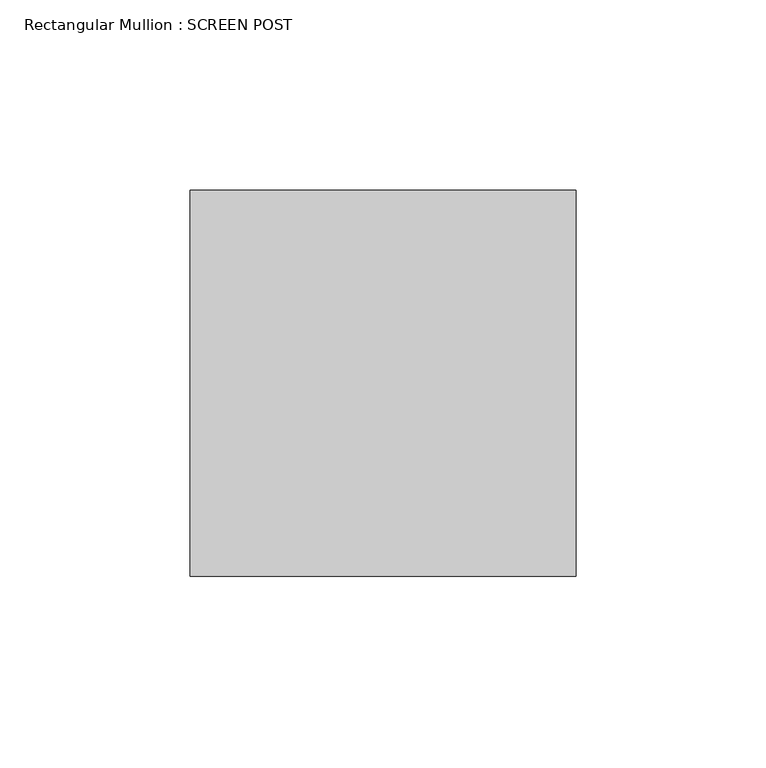
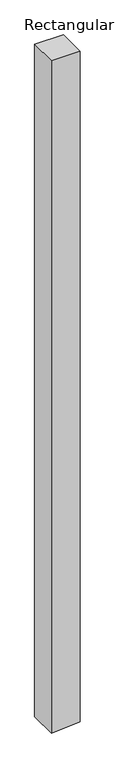
"""IFC4 building model written with IfcOpenShell, lengths in millimetres: member geometry, Rectangular Mullion : SCREEN POST."""

from ifc_helpers import new_model, si_unit, frame, origin, place, context, project, spatial, polyline, outline, extrude, source, transform, mapped, element, save


def rectangular_mullion_screen_post_35e54131(model_context):
    return source(origin(), model_context, "Body", "SweptSolid", [
        extrude(outline(polyline([(0.0, 50.8), (0.0, -50.8), (-2511.8916599, -50.8), (-2509.112762, -6.3376339), (-2505.5416599, 50.8), (0.0, 50.8)])), frame((0.0, -50.8, 0.0), z_axis=(0.0, 1.0, 0.0), x_axis=(0.0, 0.0, 1.0)), (0.0, 0.0, 1.0), 101.6),
    ])


if __name__ == "__main__":
    model = new_model("IFC4")
    model_context = context("Model", 3, world=origin())
    ifc_project = project(units=[si_unit("LENGTHUNIT", "METRE", prefix="MILLI")], contexts=[model_context])
    site = spatial("IfcSite", under=ifc_project)
    building = spatial("IfcBuilding", under=site)
    placement = place(None, origin())
    rectangular_mullion_screen_post_shape = rectangular_mullion_screen_post_35e54131(model_context)
    element("IfcMember", 1, ObjectType="Rectangular Mullion : SCREEN POST", at=placement, inside=building, context=model_context, shape_type="MappedRepresentation", body=[
        mapped(rectangular_mullion_screen_post_shape, transform((0.0, 0.0, 0.0), x_axis=(1.0, 0.0, 0.0), y_axis=(0.0, 1.0, 0.0), z_axis=(0.0, 0.0, 1.0))),
    ])
    save(model, "model.ifc")

# Revit data of these elements
# Type "Rectangular Mullion : SCREEN POST"
#   built-in parameter 1007304 = 0.333333 (stored number, unit not read)
#   built-in parameter 1007301 = 0.166667 (stored number, unit not read)
#   built-in parameter 1007300 = 0.166667 (stored number, unit not read)
# Element 1 (IfcMember, "Rectangular Mullion : SCREEN POST")
#   Materials on its faces: "SCREEN PORCH FRAMING"
# Materials
#   "SCREEN PORCH FRAMING": class "Wood", colour RGB 164 134 123, transparency 0, Description = "Pinus Echinata", Cost = 0
